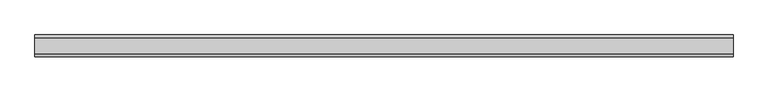
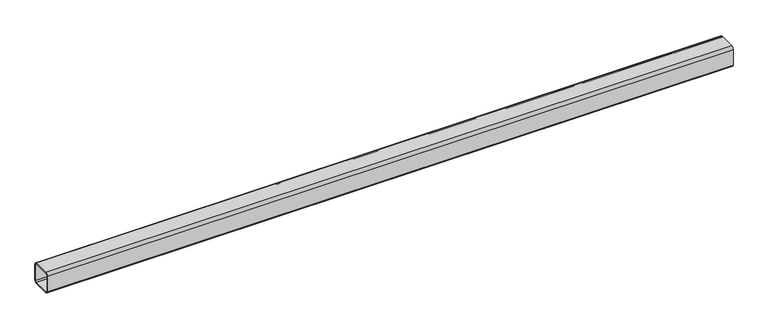
"""IFC4 building model written with IfcOpenShell, lengths in millimetres: beam geometry, Гнутый прямоугольный профиль (Трубы 30245-94) Балки : гнутый прямоуг. проф. 100x6."""

from ifc_helpers import new_model, si_unit, point, frame, frame_2d, origin, place, context, project, spatial, polyline, circle_curve, trimmed, segment, composite_curve, outline, extrude, source, transform, mapped, element, save


def beam_810e5c83(model_context):
    return source(origin(), model_context, "Body", "SweptSolid", [
        extrude(outline(composite_curve([segment(polyline([(-38.0, 50.0), (38.0, 50.0)]), True, "CONTINUOUS"), segment(trimmed(circle_curve(frame_2d((38.0, 38.0)), 12.0), [point((38.0, 50.0))], [point((50.0, 38.0))], False, "CARTESIAN"), True, "CONTINUOUS"), segment(polyline([(50.0, 38.0), (50.0, -38.0)]), True, "CONTINUOUS"), segment(trimmed(circle_curve(frame_2d((38.0, -38.0)), 12.0), [point((50.0, -38.0))], [point((38.0, -50.0))], False, "CARTESIAN"), True, "CONTINUOUS"), segment(polyline([(38.0, -50.0), (-38.0, -50.0)]), True, "CONTINUOUS"), segment(trimmed(circle_curve(frame_2d((-38.0, -38.0)), 12.0), [point((-38.0, -50.0))], [point((-50.0, -38.0))], False, "CARTESIAN"), True, "CONTINUOUS"), segment(polyline([(-50.0, -38.0), (-50.0, 38.0)]), True, "CONTINUOUS"), segment(trimmed(circle_curve(frame_2d((-38.0, 38.0)), 12.0), [point((-50.0, 38.0))], [point((-38.0, 50.0))], False, "CARTESIAN"), True, "CONTINUOUS")], self_intersect=False), holes=[composite_curve([segment(trimmed(circle_curve(frame_2d((-38.0, 38.0)), 6.0), [point((-38.0, 44.0))], [point((-44.0, 38.0))], True, "CARTESIAN"), True, "CONTINUOUS"), segment(polyline([(-44.0, 38.0), (-44.0, -38.0)]), True, "CONTINUOUS"), segment(trimmed(circle_curve(frame_2d((-38.0, -38.0)), 6.0), [point((-44.0, -38.0))], [point((-38.0, -44.0))], True, "CARTESIAN"), True, "CONTINUOUS"), segment(polyline([(-38.0, -44.0), (38.0, -44.0)]), True, "CONTINUOUS"), segment(trimmed(circle_curve(frame_2d((38.0, -38.0)), 6.0), [point((38.0, -44.0))], [point((44.0, -38.0))], True, "CARTESIAN"), True, "CONTINUOUS"), segment(polyline([(44.0, -38.0), (44.0, 38.0)]), True, "CONTINUOUS"), segment(trimmed(circle_curve(frame_2d((38.0, 38.0)), 6.0), [point((44.0, 38.0))], [point((38.0, 44.0))], True, "CARTESIAN"), True, "CONTINUOUS"), segment(polyline([(38.0, 44.0), (-38.0, 44.0)]), True, "CONTINUOUS")], self_intersect=False)]), frame((-1601.0, 0.0, 0.0), z_axis=(1.0, 0.0, 0.0), x_axis=(0.0, 1.0, 0.0)), (0.0, 0.0, 1.0), 3202.0),
    ])


if __name__ == "__main__":
    model = new_model("IFC4")
    model_context = context("Model", 3, world=origin())
    ifc_project = project(units=[si_unit("LENGTHUNIT", "METRE", prefix="MILLI")], contexts=[model_context])
    site = spatial("IfcSite", under=ifc_project)
    building = spatial("IfcBuilding", under=site)
    placement = place(None, origin())
    beam_shape = beam_810e5c83(model_context)
    element("IfcBeam", 1, ObjectType="Гнутый прямоугольный профиль (Трубы 30245-94) Балки : гнутый прямоуг. проф. 100x6", at=placement, inside=building, context=model_context, shape_type="MappedRepresentation", body=[
        mapped(beam_shape, transform((0.0, 0.0, 0.0), x_axis=(1.0, 0.0, 0.0), y_axis=(0.0, 1.0, 0.0), z_axis=(0.0, 0.0, 1.0))),
    ])
    save(model, "model.ifc")

# Revit data of these elements
# Type "Гнутый прямоугольный профиль (Трубы 30245-94) Балки : гнутый прямоуг. проф. 100x6"
#   ri = 12 mm
#   ra = 6 mm
#   W = 0.173578
#   Vz = 50 mm
#   Vy = 50 mm
#   Vpz = 50 mm
#   Vpy = 50 mm
#   Length [instance default] = 1500 mm
#   bf = 100 mm
#   d = 100 mm
#   tf = 6 mm
#   tw = 6 mm
#   A = 0.00226 m²
#   Structural Material [instance default] = Металл - Сталь - 345 МПa
#   Assembly Code = ""
# Element 1 (IfcBeam, "Гнутый прямоугольный профиль (Трубы 30245-94) Балки : гнутый прямоуг. проф. 100x6")
#   Structural Material = C235
#   Materials on its faces: "C235"
# Materials
#   "Металл - Сталь - 345 МПa": class "Металл", colour RGB 247 247 247, transparency 0
#   "C235": class "Не назначено", colour RGB 0 0 0, transparency 0
